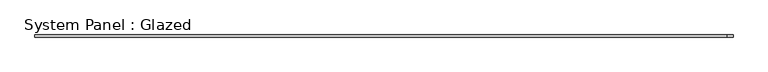
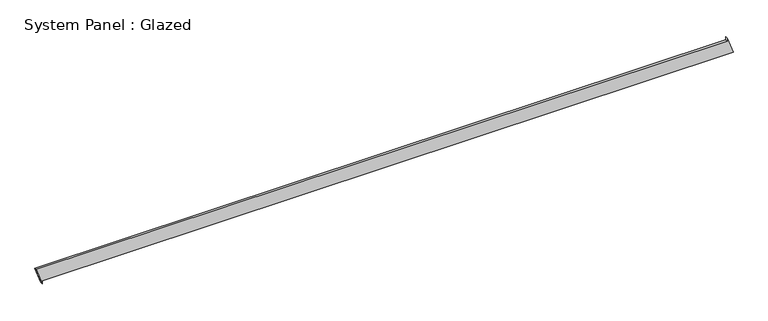
"""IFC4 building model written with IfcOpenShell, lengths in millimetres: plate geometry, System Panel : Glazed."""

from ifc_helpers import new_model, si_unit, frame, origin, place, context, project, spatial, polyline, outline, extrude, source, transform, mapped, element, save


def system_panel_glazed_5388cc54(model_context):
    return source(origin(), model_context, "Body", "SweptSolid", [
        extrude(outline(polyline([(0.0, -3957.0720499), (35.3553391, -3957.0720499), (35.3553391, 4026.9181807), (234.328916, 3957.2301733), (198.9735769, 3957.2304684), (198.9069288, -4026.9181807), (0.0, -3957.0720499)])), frame((0.0, -49.5, 0.0), z_axis=(0.0, 1.0, 0.0), x_axis=(0.0, 0.0, 1.0)), (0.0, 0.0, 1.0), 25.0),
    ])


if __name__ == "__main__":
    model = new_model("IFC4")
    model_context = context("Model", 3, world=origin())
    ifc_project = project(units=[si_unit("LENGTHUNIT", "METRE", prefix="MILLI")], contexts=[model_context])
    site = spatial("IfcSite", under=ifc_project)
    building = spatial("IfcBuilding", under=site)
    placement = place(None, origin())
    system_panel_glazed_shape = system_panel_glazed_5388cc54(model_context)
    element("IfcPlate", 1, ObjectType="System Panel : Glazed", at=placement, inside=building, context=model_context, shape_type="MappedRepresentation", body=[
        mapped(system_panel_glazed_shape, transform((0.0, 0.0, 0.0), x_axis=(1.0, 0.0, 0.0), y_axis=(0.0, 1.0, 0.0), z_axis=(0.0, 0.0, 1.0))),
    ])
    save(model, "model.ifc")

# Revit data of these elements
# Element 1 (IfcPlate, "System Panel : Glazed")
#   Materials on its faces: "Glass"
# Materials
#   "Glass": class "Glass", colour RGB 218 227 224, transparency 0.85, Description = "Soda Lime Glass", Cost = 0
